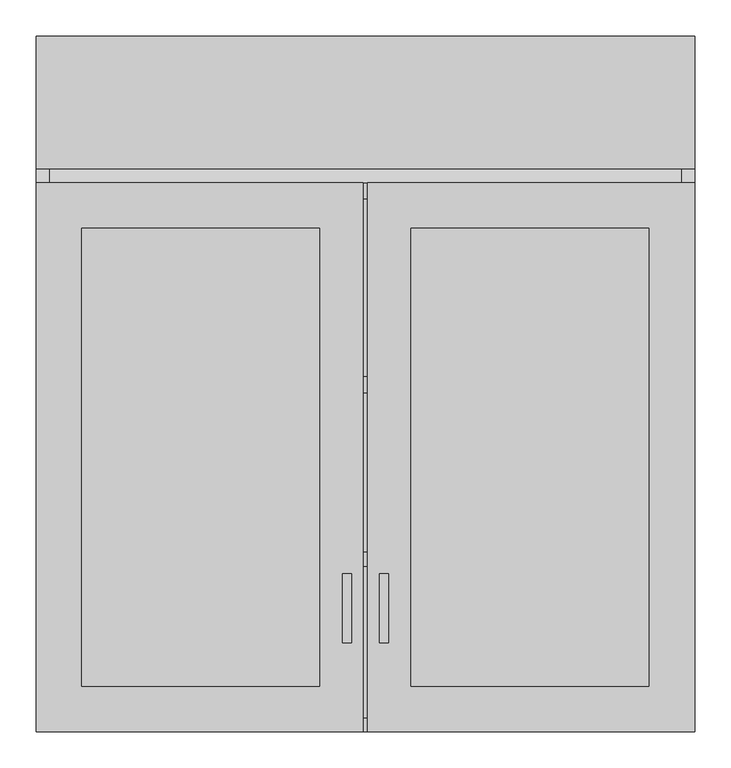
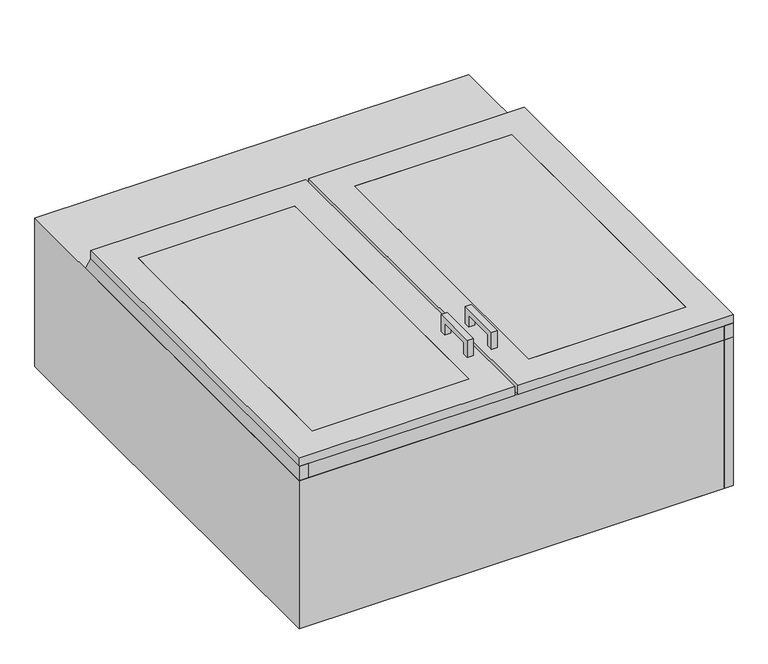
"""IFC4 building model written with IfcOpenShell, lengths in millimetres: proxy geometry, CE040 - Cabinet, W-H, 2 SH, 2 GDO, Sloping Top, 38x36x13 : CE040 - Cabinet, W-H, 2 SH, 2 GDO, Sloping Top, 38x36x13."""

from ifc_helpers import new_model, si_unit, frame, origin, origin_with_axes, place, context, project, spatial, polyline, outline, extrude, source, transform, mapped, element, save


def specialty_equipment_656b94b3(model_context):
    return source(origin(), model_context, "Body", "SweptSolid", [
        extrude(outline(polyline([(965.2, 19.05), (943.0563437, 19.05), (739.8563437, 361.95), (762.0, 361.95), (965.2, 19.05)])), frame((-438.15, 0.0, 0.0), z_axis=(1.0, 0.0, 0.0), x_axis=(0.0, 1.0, 0.0)), (0.0, 0.0, 1.0), 876.3),
        extrude(outline(polyline([(219.0655468, 419.0810937), (219.0655468, 381.0), (206.3958968, 381.0), (206.3958968, 406.4114436), (136.5230095, 406.4114436), (136.5230095, 381.0), (123.8533595, 381.0), (123.8533595, 419.0810937), (219.0655468, 419.0810937)])), frame((-31.4565288, 0.0, 0.0), z_axis=(1.0, 0.0, 0.0), x_axis=(0.0, 1.0, 0.0)), (0.0, 0.0, 1.0), 12.4023438),
        extrude(outline(polyline([(219.0655468, 419.0810937), (219.0655468, 381.0), (206.3958968, 381.0), (206.3958968, 406.4114436), (136.5230095, 406.4114436), (136.5230095, 381.0), (123.8533595, 381.0), (123.8533595, 419.0810937), (219.0655468, 419.0810937)])), frame((19.3476563, 0.0, 0.0), z_axis=(1.0, 0.0, 0.0), x_axis=(0.0, 1.0, 0.0)), (0.0, 0.0, 1.0), 12.4023438),
        extrude(outline(polyline([(457.2, 965.2), (457.2, 0.0), (-457.2, 0.0), (-457.2, 965.2), (457.2, 965.2)])), origin_with_axes(), (0.0, 0.0, 1.0), 330.2),
        extrude(outline(polyline([(762.0, 0.0), (0.0, 0.0), (0.0, 361.95), (762.0, 361.95), (965.2, 19.05), (965.2, 0.0), (762.0, 0.0)])), frame((438.15, 0.0, 0.0), z_axis=(1.0, 0.0, 0.0), x_axis=(0.0, 1.0, 0.0)), (0.0, 0.0, 1.0), 19.05),
        extrude(outline(polyline([(965.2, 0.0), (0.0, 0.0), (0.0, 361.95), (762.0, 361.95), (965.2, 19.05), (965.2, 0.0)])), frame((-457.2, 0.0, 0.0), z_axis=(1.0, 0.0, 0.0), x_axis=(0.0, 1.0, 0.0)), (0.0, 0.0, 1.0), 19.05),
        extrude(outline(polyline([(393.7, 63.5), (63.5, 63.5), (63.5, 698.5), (393.7, 698.5), (393.7, 63.5)])), frame((0.0, 0.0, 374.65), z_axis=(0.0, 0.0, 1.0), x_axis=(1.0, 0.0, 0.0)), (0.0, 0.0, 1.0), 6.35),
        extrude(outline(polyline([(-63.5, 63.5), (-393.7, 63.5), (-393.7, 698.5), (-63.5, 698.5), (-63.5, 63.5)])), frame((0.0, 0.0, 374.65), z_axis=(0.0, 0.0, 1.0), x_axis=(1.0, 0.0, 0.0)), (0.0, 0.0, 1.0), 6.35),
        extrude(outline(polyline([(457.2, 0.0), (3.175, 0.0), (3.175, 762.0), (457.2, 762.0), (457.2, 0.0)]), holes=[polyline([(393.7, 63.5), (393.7, 698.5), (63.5, 698.5), (63.5, 63.5), (393.7, 63.5)])]), frame((0.0, 0.0, 361.95), z_axis=(0.0, 0.0, 1.0), x_axis=(1.0, 0.0, 0.0)), (0.0, 0.0, 1.0), 19.05),
        extrude(outline(polyline([(438.15, 470.4491105), (-438.15, 470.4491105), (-438.15, 492.3899118), (438.15, 492.3899118), (438.15, 470.4491105)])), frame((0.0, 0.0, 19.05), z_axis=(0.0, 0.0, 1.0), x_axis=(1.0, 0.0, 0.0)), (0.0, 0.0, 1.0), 342.9),
        extrude(outline(polyline([(438.15, 229.9011198), (-438.15, 229.9011198), (-438.15, 249.0078655), (438.15, 249.0078655), (438.15, 229.9011198)])), frame((0.0, 0.0, 19.05), z_axis=(0.0, 0.0, 1.0), x_axis=(1.0, 0.0, 0.0)), (0.0, 0.0, 1.0), 342.9),
        extrude(outline(polyline([(-3.175, 0.0), (-457.2, 0.0), (-457.2, 762.0), (-3.175, 762.0), (-3.175, 0.0)]), holes=[polyline([(-63.5, 63.5), (-63.5, 698.5), (-393.7, 698.5), (-393.7, 63.5), (-63.5, 63.5)])]), frame((0.0, 0.0, 361.95), z_axis=(0.0, 0.0, 1.0), x_axis=(1.0, 0.0, 0.0)), (0.0, 0.0, 1.0), 19.05),
        extrude(outline(polyline([(438.15, 965.2), (438.15, 19.05), (-438.15, 19.05), (-438.15, 965.2), (438.15, 965.2)])), origin_with_axes(), (0.0, 0.0, 1.0), 19.05),
        extrude(outline(polyline([(-438.15, 19.05), (438.15, 19.05), (438.15, 0.0), (-438.15, 0.0), (-438.15, 19.05)])), origin_with_axes(), (0.0, 0.0, 1.0), 361.95),
    ])


if __name__ == "__main__":
    model = new_model("IFC4")
    model_context = context("Model", 3, world=origin())
    ifc_project = project(units=[si_unit("LENGTHUNIT", "METRE", prefix="MILLI")], contexts=[model_context])
    site = spatial("IfcSite", under=ifc_project)
    building = spatial("IfcBuilding", under=site)
    placement = place(None, origin())
    specialty_equipment_shape = specialty_equipment_656b94b3(model_context)
    element("IfcBuildingElementProxy", 1, Name="CE040 - Cabinet, W-H, 2 SH, 2 GDO, Sloping Top, 38x36x13 : CE040 - Cabinet, W-H, 2 SH, 2 GDO, Sloping Top, 38x36x13", ObjectType="CE040 - Cabinet, W-H, 2 SH, 2 GDO, Sloping Top, 38x36x13 : CE040 - Cabinet, W-H, 2 SH, 2 GDO, Sloping Top, 38x36x13", at=placement, inside=building, context=model_context, shape_type="MappedRepresentation", body=[
        mapped(specialty_equipment_shape, transform((0.0, 0.0, 0.0), x_axis=(1.0, 0.0, 0.0), y_axis=(0.0, 1.0, 0.0), z_axis=(0.0, 0.0, 1.0))),
    ])
    save(model, "model.ifc")

# Revit data of these elements
# Type "CE040 - Cabinet, W-H, 2 SH, 2 GDO, Sloping Top, 38x36x13 : CE040 - Cabinet, W-H, 2 SH, 2 GDO, Sloping Top, 38x36x13"
#   JSN = "CE040"
#   Nomenclature = "Cabinet, W/H, 2 SH, 2 GDO, Sloping Top, 38x36x13"
#   Utility_6 = "-"
#   Utility_5 = "-"
#   Utility_4 = "-"
#   Utility_3 = "-"
#   Utility_2 = "-"
#   Utility_1 = "-"
#   Unit_Issue = "EA"
#   Price_Date = "07/08/2010"
#   Nomenclature = "Cabinet, W/H, 2 SH, 2 GDO, Sloping Top, 38x36x13"
#   NSN = "6530"
#   Location [instance default] = ""
#   JSN_Name = "CE040"
#   Hertz_swit = "0"
#   Hertz_dep = "0"
#   Hertz = "0"
#   Desc = "Wall hung cabinet with two adjustable shelves, framed-glass hinged doors, and sloping top. Also referred to as a framed-glass hinged double door wall case. For general purpose use throughout the facility."
#   CAT_VA = "-"
#   CAT_Navy = "A"
#   CAT_IHS = "A"
#   CAT_Army = "A"
#   CAT_AF = "-"
#   BTUPerHour = "0"
#   Width_IN = 36
#   Weight_AV = 0
#   Watts2 = 0
#   Watts1 = 0
#   Volts2 = 0
#   Volts1 = 0
#   Phase2 = 0
#   Phase1 = 0
#   Height_IN = 38
#   Depth_IN = 13
#   Default Elevation = 4' - 6"
#   Amps2 = 0
#   Amps1 = 0
#   Top Panel Material = none
#   Side Panel Material = none
#   Shelf Panel Material = none
#   Door Panel Material = none
#   Door Glass Material = Glass
#   Back Panel Material = none
#   Assembly Code = ""
# Element 1 (IfcBuildingElementProxy, "CE040 - Cabinet, W-H, 2 SH, 2 GDO, Sloping Top, 38x36x13 : CE040 - Cabinet, W-H, 2 SH, 2 GDO, Sloping Top, 38x36x13")
#   Materials on its faces: "Default metal", "Glass", "EquipSpace"
# Materials
#   "Glass": class "Glass", colour RGB 0 128 192, transparency 0.75
#   "Default metal": class "Unassigned", colour RGB 204 204 204, transparency 0
#   "EquipSpace": class "Unassigned", colour RGB 221 217 195, transparency 0.5
